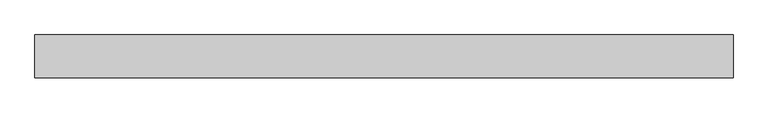
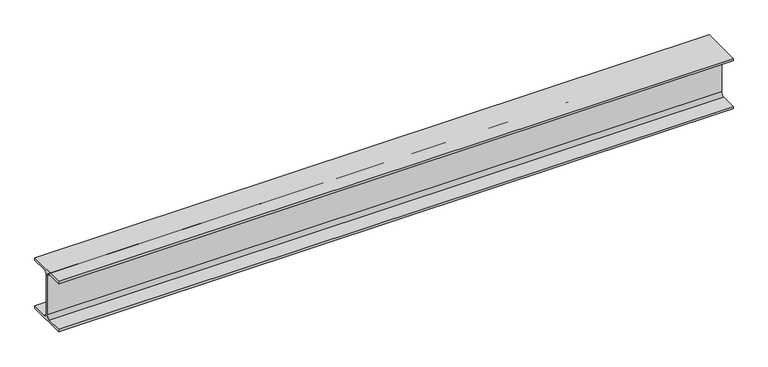
"""IFC4 building model written with IfcOpenShell, lengths in millimetres: beam geometry, 0912_Steel Framing_H-KSD3502 : H_SB_ASB_H-194x150x6x9."""

from ifc_helpers import new_model, si_unit, point, frame, frame_2d, origin, place, context, project, spatial, polyline, circle_curve, trimmed, segment, composite_curve, outline, extrude, source, transform, mapped, element, save


def beam_d8a52078(model_context):
    return source(origin(), model_context, "Body", "SweptSolid", [
        extrude(outline(composite_curve([segment(polyline([(-75.0, -88.0), (-16.0, -88.0)]), True, "CONTINUOUS"), segment(trimmed(circle_curve(frame_2d((-16.0, -75.0)), 13.0), [point((-16.0, -88.0))], [point((-3.0, -75.0))], True, "CARTESIAN"), True, "CONTINUOUS"), segment(polyline([(-3.0, -75.0), (-3.0, 75.0)]), True, "CONTINUOUS"), segment(trimmed(circle_curve(frame_2d((-16.0, 75.0)), 13.0), [point((-3.0, 75.0))], [point((-16.0, 88.0))], True, "CARTESIAN"), True, "CONTINUOUS"), segment(polyline([(-16.0, 88.0), (-75.0, 88.0), (-75.0, 97.0), (75.0, 97.0), (75.0, 88.0), (16.0, 88.0)]), True, "CONTINUOUS"), segment(trimmed(circle_curve(frame_2d((16.0, 75.0)), 13.0), [point((16.0, 88.0))], [point((3.0, 75.0))], True, "CARTESIAN"), True, "CONTINUOUS"), segment(polyline([(3.0, 75.0), (3.0, -75.0)]), True, "CONTINUOUS"), segment(trimmed(circle_curve(frame_2d((16.0, -75.0)), 13.0), [point((3.0, -75.0))], [point((16.0, -88.0))], True, "CARTESIAN"), True, "CONTINUOUS"), segment(polyline([(16.0, -88.0), (75.0, -88.0), (75.0, -97.0), (-75.0, -97.0), (-75.0, -88.0)]), True, "CONTINUOUS")], self_intersect=False)), frame((-1253.7727018, 0.0, 0.0), z_axis=(1.0, 0.0, 0.0), x_axis=(0.0, 1.0, 0.0)), (0.0, 0.0, 1.0), 2453.7727018),
    ])


if __name__ == "__main__":
    model = new_model("IFC4")
    model_context = context("Model", 3, world=origin())
    ifc_project = project(units=[si_unit("LENGTHUNIT", "METRE", prefix="MILLI")], contexts=[model_context])
    site = spatial("IfcSite", under=ifc_project)
    building = spatial("IfcBuilding", under=site)
    placement = place(None, origin())
    beam_shape = beam_d8a52078(model_context)
    element("IfcBeam", 1, ObjectType="0912_Steel Framing_H-KSD3502 : H_SB_ASB_H-194x150x6x9", at=placement, inside=building, context=model_context, shape_type="MappedRepresentation", body=[
        mapped(beam_shape, transform((0.0, 0.0, 0.0), x_axis=(1.0, 0.0, 0.0), y_axis=(0.0, 1.0, 0.0), z_axis=(0.0, 0.0, 1.0))),
    ])
    save(model, "model.ifc")

# Revit data of these elements
# Type "0912_Steel Framing_H-KSD3502 : H_SB_ASB_H-194x150x6x9"
#   H_WM Code_1 = "S01AA002-00001 | Main Steel Structure Fabrication Work | Shelter/Building | Medium Steel - Standard (90KG/M>Weight≥30KG/M) | Material: (   )"
#   H_WM Code_2 = "S03AA028-00001 | Main Steel Structure Erection Work | Shelter/Building | Medium Steel (90KG/M>Weight≥30KG/M) | Material: (   )"
#   H_WM Code_3 = "S01AA010-00001 | Main Steel Structure Fabrication Work | Shelter/Building | Steel Painting/Coating | for Non-Fireproofed Steel Surface, Surface Preparation, Primer, Second & Final Coat | Material: (   )"
#   H_Q'ty Cal Type Tag = "SB-Q2"
#   Width = 15.0 cm
#   Web Thickness = 0.6 cm
#   Web Fillet = 1.3 cm
#   Warping Constant = 43316.0 cm⁶
#   W = 0
#   Torsional Moment of Inertia = 8.622 cm⁴
#   Section Area = 39.01 cm²
#   Plastic Modulus weak axis = 104.0 cm³
#   Plastic Modulus strong axis = 309.0 cm³
#   Perimeter = 0.95 m²/m
#   Nominal Weight = 30.60 kgf/m
#   Moment of Inertia weak axis = 507.00 cm⁴
#   Moment of Inertia strong axis = 2690.00 cm⁴
#   Height = 19.4 cm
#   Flange Thickness = 0.9 cm
#   Elastic Modulus weak axis = 67.6 cm³
#   Elastic Modulus strong axis = 277.0 cm³
#   Centroid Vertical = 9.7 cm
#   Centroid Horizontal = 7.5 cm
#   Ix = 26900000
#   Length [instance default] = 1.5240 m
#   Zx = 309000
#   b = 0.1500 m
#   h = 0.1940 m
#   r = 0.0130 m
#   s = 0.0060 m
#   t = 0.0090 m
#   A = 0.003901 m²
#   Structural Material [instance default] = Steel, 45-345
#   Assembly Code = ""
# Element 1 (IfcBeam, "0912_Steel Framing_H-KSD3502 : H_SB_ASB_H-194x150x6x9")
#   Structural Material = none
# Materials
#   "Steel, 45-345": class "Metal", colour RGB 189 187 185, transparency 0, Description = "Steel 345 MPa", Cost = 0
